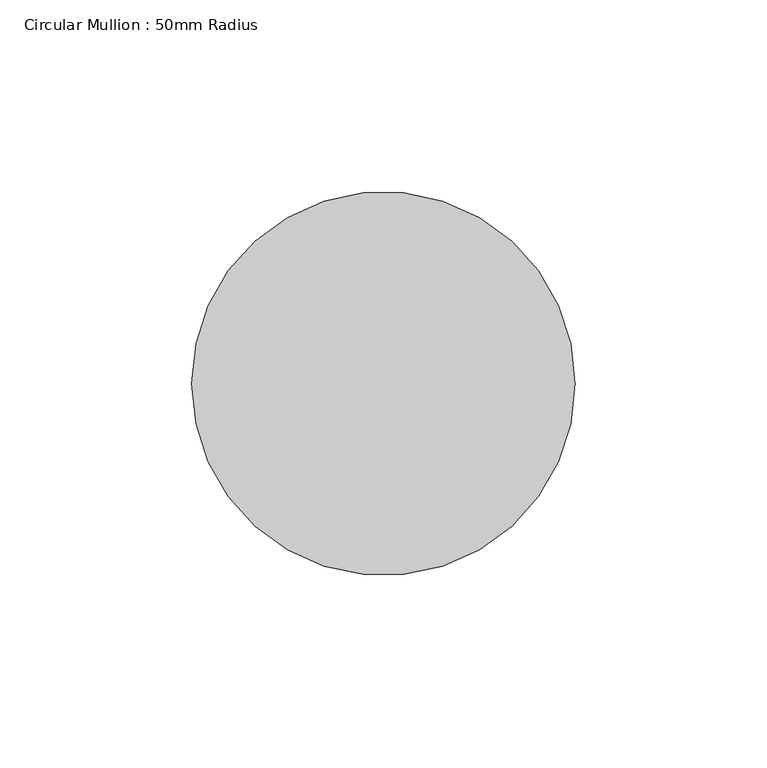
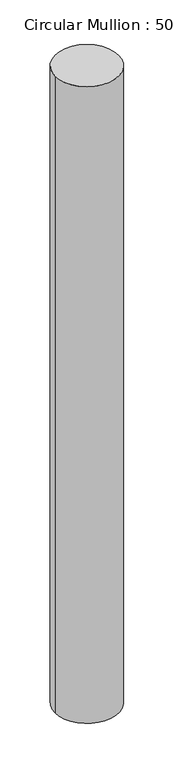
"""IFC4 building model written with IfcOpenShell, lengths in millimetres: member geometry, Circular Mullion : 50mm Radius."""

from ifc_helpers import new_model, si_unit, point, frame, origin, origin_2d, place, context, project, spatial, circle_curve, trimmed, segment, composite_curve, outline, extrude, source, transform, mapped, element, save


def circular_mullion_50mm_radius_5bc55f0f(model_context):
    return source(origin(), model_context, "Body", "SweptSolid", [
        extrude(outline(composite_curve([segment(trimmed(circle_curve(origin_2d(), 50.0), [point((50.0, 0.0))], [point((-50.0, 0.0))], False, "CARTESIAN"), True, "CONTINUOUS"), segment(trimmed(circle_curve(origin_2d(), 50.0), [point((-50.0, 0.0))], [point((50.0, 0.0))], False, "CARTESIAN"), True, "CONTINUOUS")], self_intersect=False)), frame((0.0, 0.0, -1055.9001031), z_axis=(0.0, 0.0, 1.0), x_axis=(1.0, 0.0, 0.0)), (0.0, 0.0, 1.0), 1055.9001031),
    ])


if __name__ == "__main__":
    model = new_model("IFC4")
    model_context = context("Model", 3, world=origin())
    ifc_project = project(units=[si_unit("LENGTHUNIT", "METRE", prefix="MILLI")], contexts=[model_context])
    site = spatial("IfcSite", under=ifc_project)
    building = spatial("IfcBuilding", under=site)
    placement = place(None, origin())
    circular_mullion_50mm_radius_shape = circular_mullion_50mm_radius_5bc55f0f(model_context)
    element("IfcMember", 1, ObjectType="Circular Mullion : 50mm Radius", at=placement, inside=building, context=model_context, shape_type="MappedRepresentation", body=[
        mapped(circular_mullion_50mm_radius_shape, transform((0.0, 0.0, 0.0), x_axis=(1.0, 0.0, 0.0), y_axis=(0.0, 1.0, 0.0), z_axis=(0.0, 0.0, 1.0))),
    ])
    save(model, "model.ifc")

# Revit data of these elements
# Type "Circular Mullion : 50mm Radius"
#   built-in parameter 1007350 = 0.164042 (stored number, unit not read)
# Element 1 (IfcMember, "Circular Mullion : 50mm Radius")
#   Materials on its faces: "Aluminium"
# Materials
#   "Aluminium": class "Metal", colour RGB 247 247 247, transparency 0, Description = "Aluminium 6061", Cost = 0
